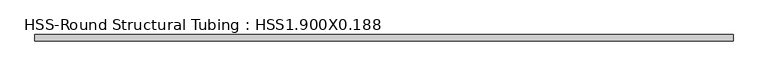
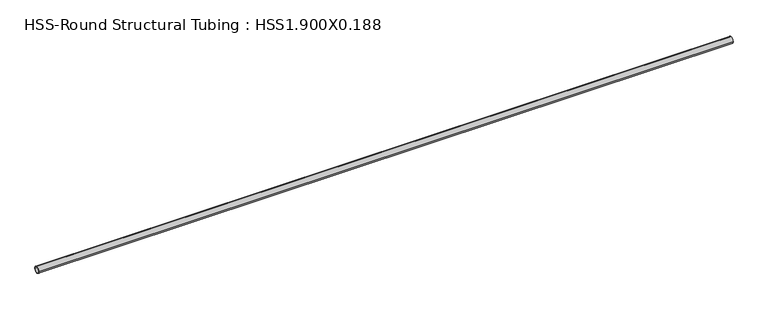
"""IFC4 building model written with IfcOpenShell, lengths in millimetres: member geometry, HSS-Round Structural Tubing : HSS1.900X0.188."""

from ifc_helpers import new_model, si_unit, point, frame, origin, origin_2d, place, context, project, spatial, circle_curve, trimmed, segment, composite_curve, outline, extrude, source, transform, mapped, element, save


def hss_round_structural_tubing_hss1_900x0_188_b26e8f7a(model_context):
    return source(origin(), model_context, "Body", "SweptSolid", [
        extrude(outline(composite_curve([segment(trimmed(circle_curve(origin_2d(), 24.13), [point((-24.13, 0.0))], [point((24.13, 0.0))], False, "CARTESIAN"), True, "CONTINUOUS"), segment(trimmed(circle_curve(origin_2d(), 24.13), [point((24.13, 0.0))], [point((-24.13, 0.0))], False, "CARTESIAN"), True, "CONTINUOUS")], self_intersect=False), holes=[composite_curve([segment(trimmed(circle_curve(origin_2d(), 19.7104), [point((19.7104, 0.0))], [point((-19.7104, 0.0))], True, "CARTESIAN"), True, "CONTINUOUS"), segment(trimmed(circle_curve(origin_2d(), 19.7104), [point((-19.7104, 0.0))], [point((19.7104, 0.0))], True, "CARTESIAN"), True, "CONTINUOUS")], self_intersect=False)]), frame((-2585.8479774, 0.0, 0.0), z_axis=(1.0, 0.0, 0.0), x_axis=(0.0, 1.0, 0.0)), (0.0, 0.0, 1.0), 5139.611762),
    ])


if __name__ == "__main__":
    model = new_model("IFC4")
    model_context = context("Model", 3, world=origin())
    ifc_project = project(units=[si_unit("LENGTHUNIT", "METRE", prefix="MILLI")], contexts=[model_context])
    site = spatial("IfcSite", under=ifc_project)
    building = spatial("IfcBuilding", under=site)
    placement = place(None, origin())
    hss_round_structural_tubing_hss1_900x0_188_shape = hss_round_structural_tubing_hss1_900x0_188_b26e8f7a(model_context)
    element("IfcMember", 1, ObjectType="HSS-Round Structural Tubing : HSS1.900X0.188", at=placement, inside=building, context=model_context, shape_type="MappedRepresentation", body=[
        mapped(hss_round_structural_tubing_hss1_900x0_188_shape, transform((0.0, 0.0, 0.0), x_axis=(1.0, 0.0, 0.0), y_axis=(0.0, 1.0, 0.0), z_axis=(0.0, 0.0, 1.0))),
    ])
    save(model, "model.ifc")

# Revit data of these elements
# Type "HSS-Round Structural Tubing : HSS1.900X0.188"
#   Assembly Code = "B10"
#   t = 4.42 mm
#   W = 3.44
#   Length [instance default] = 1524 mm
#   OD = 48.26 mm
#   A = 0.000608386 m²
#   Structural Material [instance default] = Steel ASTM A500, Grade B, Round
# Element 1 (IfcMember, "HSS-Round Structural Tubing : HSS1.900X0.188")
#   Materials on its faces: "Steel ASTM A500, Grade B, Round"
# Materials
#   "Steel ASTM A500, Grade B, Round": class "Metal", colour RGB 199 199 199, transparency 0, Description = "Carbon steel", Cost = 0
